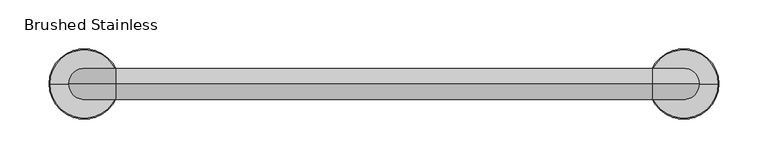
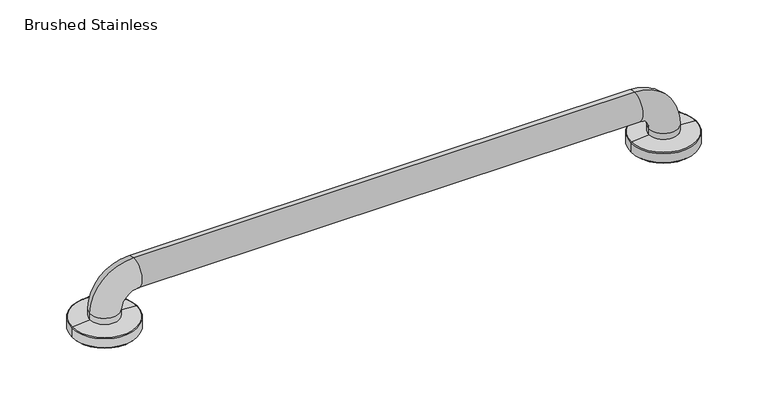
"""IFC4 building model written with IfcOpenShell, lengths in millimetres: furniture geometry, Grab_Bar-Kohler-Contemporary_K1456X : Brushed Stainless."""

import ifcopenshell
import ifcopenshell.guid

model = None  # the IFC model being written
_history = None  # IfcOwnerHistory: only IFC2X3 demands one
_inside = {}  # id of a spatial element -> (the spatial element, [elements in it])
_under = {}  # id of a project, library or spatial element -> (it, [spatial elements below it])
_declared = {}  # id of a project -> (the project, [libraries it declares])
_typed = {}  # id of a type object -> (the type object, [elements of that type])
_made_of = {}  # id of a material, layer set ... -> (it, [elements and type objects made of it])


def new_model(schema):
    """Start an empty IFC model of exactly this schema.

    Asked for "IFC4X3", IfcOpenShell would pick the latest addendum, in which some entities
    have other attributes; the version numbers below select the first issue.
    IFC2X3 requires an IfcOwnerHistory on every rooted entity: one is made here for all.
    """
    global model, _history
    if schema == "IFC4X3":
        model = ifcopenshell.file(schema_version=(4, 3, 0, 0))
    else:
        model = ifcopenshell.file(schema=schema)
    _inside.clear()
    _under.clear()
    _declared.clear()
    _typed.clear()
    _made_of.clear()
    _history = None
    if model.schema == "IFC2X3":
        org = make("IfcOrganization", Name="unknown")
        user = make(
            "IfcPersonAndOrganization",
            ThePerson=make("IfcPerson", FamilyName="unknown"),
            TheOrganization=org,
        )
        app = make(
            "IfcApplication",
            ApplicationDeveloper=org,
            Version="unknown",
            ApplicationFullName="unknown",
            ApplicationIdentifier="unknown",
        )
        _history = make(
            "IfcOwnerHistory",
            OwningUser=user,
            OwningApplication=app,
            ChangeAction="ADDED",
            CreationDate=0,
        )
    return model


def make(cls, **values):
    """One entity of the class cls with the attributes given. An attribute that is None is left unset."""
    return model.create_entity(
        cls, **{name: value for name, value in values.items() if value is not None}
    )


def rooted(cls, **values):
    """An entity with a GlobalId (a new one), such as an element, a storey or a relation."""
    return make(cls, GlobalId=ifcopenshell.guid.new(), OwnerHistory=_history, **values)


def si_unit(unit_type, name, prefix=None):
    """IfcSIUnit, for example si_unit("LENGTHUNIT", "METRE", prefix="MILLI")."""
    return make("IfcSIUnit", UnitType=unit_type, Prefix=prefix, Name=name)


def assignment(units):
    """IfcUnitAssignment: the units of a project."""
    return None if units is None else make("IfcUnitAssignment", Units=units)


def point(xyz):
    """IfcCartesianPoint."""
    return None if xyz is None else make("IfcCartesianPoint", Coordinates=xyz)


def direction(xyz):
    """IfcDirection."""
    return None if xyz is None else make("IfcDirection", DirectionRatios=xyz)


def frame(location, z_axis=None, x_axis=None):
    """IfcAxis2Placement3D, a coordinate frame: its origin and axes. An axis left out is left unset."""
    return make(
        "IfcAxis2Placement3D",
        Location=point(location),
        Axis=direction(z_axis),
        RefDirection=direction(x_axis),
    )


def origin():
    """The frame at (0, 0, 0) with its axes left unset."""
    return frame((0.0, 0.0, 0.0))


def place(relative_to, where):
    """IfcLocalPlacement: puts the frame where relative to a parent placement (None: the world)."""
    return make(
        "IfcLocalPlacement", PlacementRelTo=relative_to, RelativePlacement=where
    )


def context(
    kind, dimensions, precision=None, world=None, true_north=None, identifier=None
):
    """IfcGeometricRepresentationContext, for example the 3D "Model" context."""
    return make(
        "IfcGeometricRepresentationContext",
        ContextIdentifier=identifier,
        ContextType=kind,
        CoordinateSpaceDimension=dimensions,
        Precision=precision,
        WorldCoordinateSystem=world,
        TrueNorth=true_north,
    )


def project(units=None, contexts=None):
    """IfcProject with its units and contexts."""
    return rooted(
        "IfcProject",
        Name="project",
        RepresentationContexts=contexts,
        UnitsInContext=assignment(units),
    )


def spatial(cls, under=None, at=None, **own):
    """A site, building, storey or space (cls), placed at a placement, below another one or the project."""
    s = rooted(cls, ObjectPlacement=at, **own)
    if under is not None:
        _under.setdefault(under.id(), (under, []))[1].append(s)
    return s


def polyline(points):
    """IfcPolyline through the points."""
    return make("IfcPolyline", Points=[point(p) for p in points])


def circle_curve(where, radius):
    """IfcCircle in the frame where."""
    return make("IfcCircle", Position=where, Radius=radius)


def ellipse_curve(where, semi_axis1, semi_axis2):
    """IfcEllipse in the frame where."""
    return make(
        "IfcEllipse", Position=where, SemiAxis1=semi_axis1, SemiAxis2=semi_axis2
    )


def trimmed(basis, trim1, trim2, sense, master):
    """IfcTrimmedCurve: the piece of a basis curve between two trims."""
    return make(
        "IfcTrimmedCurve",
        BasisCurve=basis,
        Trim1=trim1,
        Trim2=trim2,
        SenseAgreement=sense,
        MasterRepresentation=master,
    )


def shape(context_of_items, identifier, shape_type, items):
    """IfcShapeRepresentation: the items that make up one representation, for example the "Body"."""
    return make(
        "IfcShapeRepresentation",
        ContextOfItems=context_of_items,
        RepresentationIdentifier=identifier,
        RepresentationType=shape_type,
        Items=items,
    )


def source(mapping_origin, context_of_items, identifier, shape_type, items):
    """IfcRepresentationMap: a shape defined once, which mapped items show again and again."""
    return make(
        "IfcRepresentationMap",
        MappingOrigin=mapping_origin,
        MappedRepresentation=shape(context_of_items, identifier, shape_type, items),
    )


def transform(
    local_origin,
    x_axis=None,
    y_axis=None,
    z_axis=None,
    scale=None,
    scale2=None,
    scale3=None,
    uniform=True,
):
    """IfcCartesianTransformationOperator3D, or its non-uniform kind. x_axis, y_axis, z_axis: its Axis1, 2, 3."""
    if uniform:
        return make(
            "IfcCartesianTransformationOperator3D",
            Axis1=direction(x_axis),
            Axis2=direction(y_axis),
            LocalOrigin=point(local_origin),
            Scale=scale,
            Axis3=direction(z_axis),
        )
    return make(
        "IfcCartesianTransformationOperator3DnonUniform",
        Axis1=direction(x_axis),
        Axis2=direction(y_axis),
        LocalOrigin=point(local_origin),
        Scale=scale,
        Axis3=direction(z_axis),
        Scale2=scale2,
        Scale3=scale3,
    )


def mapped(mapping_source, mapping_target):
    """IfcMappedItem: shows the shape of a source again, moved by a transform."""
    return make(
        "IfcMappedItem", MappingSource=mapping_source, MappingTarget=mapping_target
    )


def made_of(thing, what):
    """Note that an element or type object is made of a material, layer set ...; save() writes the relation."""
    if what is not None:
        _made_of.setdefault(what.id(), (what, []))[1].append(thing)
    return thing


def element(
    cls,
    number,
    at=None,
    inside=None,
    cuts=None,
    type_object=None,
    material=None,
    context=None,
    identifier="Body",
    shape_type=None,
    held_by="IfcProductDefinitionShape",
    body=None,
    shapes=None,
    **own,
):
    """One element of the class cls, such as IfcWall. Its Tag is "e" and its number.

    at: its placement. inside: the storey or other place that contains it. cuts: it is an
    opening in that element (IfcRelVoidsElement). A single representation is given by context,
    identifier, shape_type and body (its items); several are given by shapes. held_by: the class
    of the entity that holds the representations. save() writes the other relations.
    """
    e = rooted(cls, Tag="e%d" % number, ObjectPlacement=at, **own)
    if body is not None:
        shapes = [shape(context, identifier, shape_type, body)]
    if shapes is not None:
        e.Representation = make(held_by, Representations=shapes)
    if inside is not None:
        _inside.setdefault(inside.id(), (inside, []))[1].append(e)
    if cuts is not None:
        rooted(
            "IfcRelVoidsElement", RelatingBuildingElement=cuts, RelatedOpeningElement=e
        )
    if type_object is not None:
        _typed.setdefault(type_object.id(), (type_object, []))[1].append(e)
    return made_of(e, material)


def aggregate(whole, parts):
    """IfcRelAggregates: a whole, such as a stair, and the parts it consists of."""
    return rooted("IfcRelAggregates", RelatingObject=whole, RelatedObjects=parts)


def save(model, path):
    """Write the relations noted so far, then the file.

    IfcRelAggregates (storeys below a building ...), IfcRelContainedInSpatialStructure (elements
    in a storey), IfcRelDefinesByType, IfcRelAssociatesMaterial and IfcRelDeclares: one each for
    every whole, place, type object, material and project.
    """
    for whole, parts in _under.values():
        aggregate(whole, parts)
    for where, things in _inside.values():
        rooted(
            "IfcRelContainedInSpatialStructure",
            RelatedElements=things,
            RelatingStructure=where,
        )
    for kind, things in _typed.values():
        rooted("IfcRelDefinesByType", RelatedObjects=things, RelatingType=kind)
    for what, things in _made_of.values():
        rooted("IfcRelAssociatesMaterial", RelatedObjects=things, RelatingMaterial=what)
    for by, libraries in _declared.values():
        rooted("IfcRelDeclares", RelatingContext=by, RelatedDefinitions=libraries)
    model.write(path)


def plane_surface(at):
    """IfcPlane: the flat surface through the origin of the frame at, square to its z axis."""
    return make("IfcPlane", Position=at)


def cylinder_surface(at, radius):
    """IfcCylindricalSurface: all points at the distance radius from the z axis of the frame at."""
    return make("IfcCylindricalSurface", Position=at, Radius=radius)


def revolved_surface(curve, axis_point, axis_direction):
    """IfcSurfaceOfRevolution: the curve turned about the line through axis_point along axis_direction."""
    return make(
        "IfcSurfaceOfRevolution",
        SweptCurve=make("IfcArbitraryOpenProfileDef", ProfileType="CURVE", Curve=curve),
        AxisPosition=make("IfcAxis1Placement", Location=point(axis_point), Axis=direction(axis_direction)),
    )


def advanced_brep(points, edges, surfaces, faces):
    """IfcAdvancedBrep: a solid bounded by faces that lie on surfaces and meet in shared edges.

    An edge is (start, end): straight between two places in points (the first is 0);
    or (start, end, curve); or (start, end, curve, False) where it runs against its curve.
    A face is (place in surfaces, loops), or (place, loops, False) where it looks against
    its surface's normal. A loop lists edges by number (the first is 1), with a minus sign
    where the edge is run from its end to its start. The first loop is the outer one.
    """
    corners = [point(p) for p in points]
    vertices = [make("IfcVertexPoint", VertexGeometry=c) for c in corners]
    made = []
    for start, end, *more in edges:
        made.append(
            make(
                "IfcEdgeCurve",
                EdgeStart=vertices[start],
                EdgeEnd=vertices[end],
                EdgeGeometry=more[0] if more else make("IfcPolyline", Points=[corners[start], corners[end]]),
                SameSense=more[1] if len(more) > 1 else True,
            )
        )
    hull = []
    for where, loops, *sense in faces:
        bounds = []
        for j, loop in enumerate(loops):
            ring = [make("IfcOrientedEdge", EdgeElement=made[abs(k) - 1], Orientation=k > 0) for k in loop]
            bounds.append(
                make(
                    "IfcFaceOuterBound" if j == 0 else "IfcFaceBound",
                    Bound=make("IfcEdgeLoop", EdgeList=ring),
                    Orientation=True,
                )
            )
        hull.append(make("IfcAdvancedFace", Bounds=bounds, FaceSurface=surfaces[where], SameSense=sense[0] if sense else True))
    return make("IfcAdvancedBrep", Outer=make("IfcClosedShell", CfsFaces=hull))


def brushed_stainless_1e49a3ae(model_context):
    return source(origin(), model_context, "Body", "AdvancedBrep", [
        advanced_brep(
        [(288.925, 0.0, 15.08125), (320.675, 0.0, 15.08125), (339.5910439, 0.0, 13.5506193), (270.0089561, 0.0, 13.5506193), (288.925, 0.0, 0.0), (320.675, 0.0, 0.0), (271.45615, 0.0, 0.0), (338.14385, 0.0, 0.0), (269.0749, 0.0, 2.38125), (340.5251, 0.0, 2.38125), (269.0749, 0.0, 12.5379293), (340.5251, 0.0, 12.5379293)],
        [
            (0, 1, circle_curve(frame((304.8, 0.0, 15.08125), z_axis=(0.0, 0.0, -1.0), x_axis=(1.0, 0.0, 0.0)), 15.875)),
            (1, 2),
            (2, 3, circle_curve(frame((304.8, 0.0, 13.5506193), z_axis=(0.0, 0.0, 1.0), x_axis=(1.0, 0.0, 0.0)), 34.7910439)),
            (3, 0),
            (1, 0, circle_curve(frame((304.8, 0.0, 15.08125), z_axis=(0.0, 0.0, -1.0), x_axis=(1.0, 0.0, 0.0)), 15.875)),
            (3, 2, circle_curve(frame((304.8, 0.0, 13.5506193), z_axis=(0.0, 0.0, 1.0), x_axis=(1.0, 0.0, 0.0)), 34.7910439)),
            (4, 5, circle_curve(frame((304.8, 0.0, 0.0), z_axis=(0.0, 0.0, -1.0), x_axis=(1.0, 0.0, 0.0)), 15.875)),
            (5, 1),
            (0, 4),
            (5, 4, circle_curve(frame((304.8, 0.0, 0.0), z_axis=(0.0, 0.0, -1.0), x_axis=(1.0, 0.0, 0.0)), 15.875)),
            (6, 7, circle_curve(frame((304.8, 0.0, 0.0), z_axis=(0.0, 0.0, -1.0), x_axis=(1.0, 0.0, 0.0)), 33.34385)),
            (7, 5),
            (4, 6),
            (7, 6, circle_curve(frame((304.8, 0.0, 0.0), z_axis=(0.0, 0.0, -1.0), x_axis=(1.0, 0.0, 0.0)), 33.34385)),
            (8, 9, circle_curve(frame((304.8, 0.0, 2.38125), z_axis=(0.0, 0.0, -1.0), x_axis=(1.0, 0.0, 0.0)), 35.7251)),
            (9, 7),
            (6, 8),
            (9, 8, circle_curve(frame((304.8, 0.0, 2.38125), z_axis=(0.0, 0.0, -1.0), x_axis=(1.0, 0.0, 0.0)), 35.7251)),
            (10, 11, circle_curve(frame((304.8, 0.0, 12.5379293), z_axis=(0.0, 0.0, -1.0), x_axis=(1.0, 0.0, 0.0)), 35.7251)),
            (11, 9),
            (8, 10),
            (11, 10, circle_curve(frame((304.8, 0.0, 12.5379293), z_axis=(0.0, 0.0, -1.0), x_axis=(1.0, 0.0, 0.0)), 35.7251)),
            (2, 11, circle_curve(frame((339.5091, 0.0, 12.5379293), z_axis=(0.0, 1.0, 0.0), x_axis=(1.0, 0.0, 0.0)), 1.016)),
            (10, 3, circle_curve(frame((270.0909, 0.0, 12.5379293), z_axis=(0.0, 1.0, 0.0), x_axis=(-1.0, 0.0, 0.0)), 1.016)),
        ],
        [
            revolved_surface(polyline([(339.5910439, 0.0, 13.5506193), (320.675, 0.0, 15.08125)]), (304.8, 0.0, 136.525), (0.0, 0.0, 1.0)),
            revolved_surface(polyline([(320.675, 0.0, 15.081249999999997), (320.675, 0.0, 0.0)]), (304.8, 0.0, 136.525), (0.0, 0.0, 1.0)),
            plane_surface(frame((304.8, 0.0, 0.0), z_axis=(0.0, 0.0, -1.0), x_axis=(1.0, 0.0, 0.0))),
            revolved_surface(polyline([(338.14385, 0.0, 0.0), (340.5251, 0.0, 2.38125)]), (304.8, 0.0, 136.525), (0.0, 0.0, 1.0)),
            cylinder_surface(frame((304.8, 0.0, 136.525), z_axis=(0.0, 0.0, 1.0), x_axis=(1.0, 0.0, 0.0)), 35.7251),
            revolved_surface(trimmed(ellipse_curve(frame((339.5091, 0.0, 12.5379293), z_axis=(0.0, -1.0, 0.0), x_axis=(1.0, 0.0, 0.0)), 1.016, 1.016), [point((340.5251, 0.0, 12.5379293))], [point((339.5910439, 0.0, 13.5506193))], True, "CARTESIAN"), (304.8, 0.0, 136.525), (0.0, 0.0, 1.0)),
        ],
        [
            (0, [[1, 2, 3, 4]]),
            (0, [[5, -4, 6, -2]]),
            (1, [[7, 8, -1, 9]]),
            (1, [[10, -9, -5, -8]]),
            (2, [[11, 12, -7, 13]]),
            (2, [[14, -13, -10, -12]]),
            (3, [[15, 16, -11, 17]]),
            (3, [[18, -17, -14, -16]]),
            (4, [[19, 20, -15, 21]]),
            (4, [[22, -21, -18, -20]]),
            (5, [[-3, 23, -19, 24]]),
            (5, [[-6, -24, -22, -23]]),
        ],
    ),
        advanced_brep(
        [(-270.0089561, 0.0, 13.5506193), (-339.5910439, 0.0, 13.5506193), (-320.675, 0.0, 15.08125), (-288.925, 0.0, 15.08125), (-269.0749, 0.0, 2.38125), (-340.5251, 0.0, 2.38125), (-340.5251, 0.0, 12.5379293), (-269.0749, 0.0, 12.5379293), (-271.45615, 0.0, 0.0), (-338.14385, 0.0, 0.0), (-288.925, 0.0, 0.0), (-320.675, 0.0, 0.0)],
        [
            (0, 1, circle_curve(frame((-304.8, 0.0, 13.5506193), z_axis=(0.0, 0.0, 1.0), x_axis=(-1.0, 0.0, 0.0)), 34.7910439)),
            (1, 2),
            (2, 3, circle_curve(frame((-304.8, 0.0, 15.08125), z_axis=(0.0, 0.0, -1.0), x_axis=(-1.0, 0.0, 0.0)), 15.875)),
            (3, 0),
            (1, 0, circle_curve(frame((-304.8, 0.0, 13.5506193), z_axis=(0.0, 0.0, 1.0), x_axis=(-1.0, 0.0, 0.0)), 34.7910439)),
            (3, 2, circle_curve(frame((-304.8, 0.0, 15.08125), z_axis=(0.0, 0.0, -1.0), x_axis=(-1.0, 0.0, 0.0)), 15.875)),
            (4, 5, circle_curve(frame((-304.8, 0.0, 2.38125), z_axis=(0.0, 0.0, 1.0), x_axis=(-1.0, 0.0, 0.0)), 35.7251)),
            (5, 6),
            (6, 7, circle_curve(frame((-304.8, 0.0, 12.5379293), z_axis=(0.0, 0.0, -1.0), x_axis=(-1.0, 0.0, 0.0)), 35.7251)),
            (7, 4),
            (5, 4, circle_curve(frame((-304.8, 0.0, 2.38125), z_axis=(0.0, 0.0, 1.0), x_axis=(-1.0, 0.0, 0.0)), 35.7251)),
            (7, 6, circle_curve(frame((-304.8, 0.0, 12.5379293), z_axis=(0.0, 0.0, -1.0), x_axis=(-1.0, 0.0, 0.0)), 35.7251)),
            (8, 9, circle_curve(frame((-304.8, 0.0, 0.0), z_axis=(0.0, 0.0, 1.0), x_axis=(-1.0, 0.0, 0.0)), 33.34385)),
            (9, 5),
            (4, 8),
            (9, 8, circle_curve(frame((-304.8, 0.0, 0.0), z_axis=(0.0, 0.0, 1.0), x_axis=(-1.0, 0.0, 0.0)), 33.34385)),
            (10, 11, circle_curve(frame((-304.8, 0.0, 0.0), z_axis=(0.0, 0.0, 1.0), x_axis=(-1.0, 0.0, 0.0)), 15.875)),
            (11, 9),
            (8, 10),
            (11, 10, circle_curve(frame((-304.8, 0.0, 0.0), z_axis=(0.0, 0.0, 1.0), x_axis=(-1.0, 0.0, 0.0)), 15.875)),
            (2, 11),
            (10, 3),
            (6, 1, circle_curve(frame((-339.5091, 0.0, 12.5379293), z_axis=(0.0, 1.0, 0.0), x_axis=(1.0, 0.0, 0.0)), 1.016)),
            (0, 7, circle_curve(frame((-270.0909, 0.0, 12.5379293), z_axis=(0.0, 1.0, 0.0), x_axis=(-1.0, 0.0, 0.0)), 1.016)),
        ],
        [
            revolved_surface(polyline([(-320.675, 0.0, 15.08125), (-339.5910439, 0.0, 13.5506193)]), (-304.8, 0.0, 70.0128086), (0.0, 0.0, -1.0)),
            cylinder_surface(frame((-304.8, 0.0, 70.0128086), z_axis=(0.0, 0.0, -1.0), x_axis=(-1.0, 0.0, 0.0)), 35.7251),
            revolved_surface(polyline([(-340.5251, 0.0, 2.38125), (-338.14385, 0.0, 0.0)]), (-304.8, 0.0, 70.0128086), (0.0, 0.0, -1.0)),
            plane_surface(frame((-304.8, 0.0, 0.0), z_axis=(0.0, 0.0, -1.0), x_axis=(-1.0, 0.0, 0.0))),
            revolved_surface(polyline([(-320.675, 0.0, 0.0), (-320.675, 0.0, 15.081249999999997)]), (-304.8, 0.0, 70.0128086), (0.0, 0.0, -1.0)),
            revolved_surface(trimmed(ellipse_curve(frame((-339.5091, 0.0, 12.5379293), z_axis=(0.0, -1.0, 0.0), x_axis=(1.0, 0.0, 0.0)), 1.016, 1.016), [point((-339.5910439, 0.0, 13.5506193))], [point((-340.5251, 0.0, 12.5379293))], True, "CARTESIAN"), (-304.8, 0.0, 70.0128086), (0.0, 0.0, -1.0)),
        ],
        [
            (0, [[1, 2, 3, 4]]),
            (0, [[5, -4, 6, -2]]),
            (1, [[7, 8, 9, 10]]),
            (1, [[11, -10, 12, -8]]),
            (2, [[13, 14, -7, 15]]),
            (2, [[16, -15, -11, -14]]),
            (3, [[17, 18, -13, 19]]),
            (3, [[20, -19, -16, -18]]),
            (4, [[-3, 21, -17, 22]]),
            (4, [[-6, -22, -20, -21]]),
            (5, [[-9, 23, -1, 24]]),
            (5, [[-12, -24, -5, -23]]),
        ],
    ),
        advanced_brep(
        [(-288.925, 0.0, 0.0), (-320.675, 0.0, 0.0), (-288.925, 0.0, 22.225), (-320.675, 0.0, 22.225), (-273.05, 0.0, 69.85), (-273.05, 0.0, 38.1), (273.05, 0.0, 38.1), (273.05, 0.0, 69.85), (320.675, 0.0, 22.225), (288.925, 0.0, 22.225), (288.925, 0.0, 0.0), (320.675, 0.0, 0.0)],
        [
            (0, 1, circle_curve(frame((-304.8, 0.0, 0.0), z_axis=(0.0, 0.0, -1.0), x_axis=(-1.0, 0.0, 0.0)), 15.875)),
            (1, 0, circle_curve(frame((-304.8, 0.0, 0.0), z_axis=(0.0, 0.0, -1.0), x_axis=(-1.0, 0.0, 0.0)), 15.875)),
            (0, 2),
            (2, 3, circle_curve(frame((-304.8, 0.0, 22.225), z_axis=(0.0, 0.0, -1.0), x_axis=(-1.0, 0.0, 0.0)), 15.875)),
            (3, 1),
            (3, 2, circle_curve(frame((-304.8, 0.0, 22.225), z_axis=(0.0, 0.0, -1.0), x_axis=(-1.0, 0.0, 0.0)), 15.875)),
            (4, 3, circle_curve(frame((-273.05, 0.0, 22.225), z_axis=(0.0, -1.0, 0.0), x_axis=(-1.0, 0.0, 0.0)), 47.625)),
            (2, 5, circle_curve(frame((-273.05, 0.0, 22.225), z_axis=(0.0, 1.0, 0.0), x_axis=(-1.0, 0.0, 0.0)), 15.875)),
            (5, 4, circle_curve(frame((-273.05, 0.0, 53.975), z_axis=(-1.0, 0.0, 0.0), x_axis=(0.0, 0.0, 1.0)), 15.875)),
            (4, 5, circle_curve(frame((-273.05, 0.0, 53.975), z_axis=(-1.0, 0.0, 0.0), x_axis=(0.0, 0.0, 1.0)), 15.875)),
            (5, 6),
            (6, 7, circle_curve(frame((273.05, 0.0, 53.975), z_axis=(-1.0, 0.0, 0.0), x_axis=(0.0, 0.0, 1.0)), 15.875)),
            (7, 4),
            (7, 6, circle_curve(frame((273.05, 0.0, 53.975), z_axis=(-1.0, 0.0, 0.0), x_axis=(0.0, 0.0, 1.0)), 15.875)),
            (8, 7, circle_curve(frame((273.05, 0.0, 22.225), z_axis=(0.0, -1.0, 0.0), x_axis=(0.0, 0.0, 1.0)), 47.625)),
            (6, 9, circle_curve(frame((273.05, 0.0, 22.225), z_axis=(0.0, 1.0, 0.0), x_axis=(0.0, 0.0, 1.0)), 15.875)),
            (9, 8, circle_curve(frame((304.8, 0.0, 22.225), z_axis=(0.0, 0.0, 1.0), x_axis=(1.0, 0.0, 0.0)), 15.875)),
            (8, 9, circle_curve(frame((304.8, 0.0, 22.225), z_axis=(0.0, 0.0, 1.0), x_axis=(1.0, 0.0, 0.0)), 15.875)),
            (10, 11, circle_curve(frame((304.8, 0.0, 0.0), z_axis=(0.0, 0.0, -1.0), x_axis=(1.0, 0.0, 0.0)), 15.875)),
            (11, 10, circle_curve(frame((304.8, 0.0, 0.0), z_axis=(0.0, 0.0, -1.0), x_axis=(1.0, 0.0, 0.0)), 15.875)),
            (9, 10),
            (11, 8),
        ],
        [
            plane_surface(frame((-304.8, 0.0, 0.0), z_axis=(0.0, 0.0, -1.0), x_axis=(0.0, -1.0, 0.0))),
            cylinder_surface(frame((-304.8, 0.0, 0.0), z_axis=(0.0, 0.0, -1.0), x_axis=(-1.0, 0.0, 0.0)), 15.875),
            revolved_surface(trimmed(ellipse_curve(frame((-304.8, 0.0, 22.225), z_axis=(0.0, 0.0, -1.0), x_axis=(-1.0, 0.0, 0.0)), 15.875, 15.875), [point((-288.925, 0.0, 22.225))], [point((-320.675, 0.0, 22.225))], True, "CARTESIAN"), (-273.05, 0.0, 22.225), (0.0, 1.0, 0.0)),
            revolved_surface(trimmed(ellipse_curve(frame((-304.8, 0.0, 22.225), z_axis=(0.0, 0.0, -1.0), x_axis=(-1.0, 0.0, 0.0)), 15.875, 15.875), [point((-320.675, 0.0, 22.225))], [point((-288.925, 0.0, 22.225))], True, "CARTESIAN"), (-273.05, 0.0, 22.225), (0.0, 1.0, 0.0)),
            cylinder_surface(frame((-273.05, 0.0, 53.975), z_axis=(-1.0, 0.0, 0.0), x_axis=(0.0, 0.0, 1.0)), 15.875),
            revolved_surface(trimmed(ellipse_curve(frame((273.05, 0.0, 53.975), z_axis=(-1.0, 0.0, 0.0), x_axis=(0.0, 0.0, 1.0)), 15.875, 15.875), [point((273.05, 0.0, 38.1))], [point((273.05, 0.0, 69.85))], True, "CARTESIAN"), (273.05, 0.0, 22.225), (0.0, 1.0, 0.0)),
            revolved_surface(trimmed(ellipse_curve(frame((273.05, 0.0, 53.975), z_axis=(-1.0, 0.0, 0.0), x_axis=(0.0, 0.0, 1.0)), 15.875, 15.875), [point((273.05, 0.0, 69.85))], [point((273.05, 0.0, 38.1))], True, "CARTESIAN"), (273.05, 0.0, 22.225), (0.0, 1.0, 0.0)),
            plane_surface(frame((304.8, 0.0, 0.0), z_axis=(0.0, 0.0, -1.0), x_axis=(0.0, -1.0, 0.0))),
            cylinder_surface(frame((304.8, 0.0, 22.225), z_axis=(0.0, 0.0, 1.0), x_axis=(1.0, 0.0, 0.0)), 15.875),
        ],
        [
            (0, [[1, 2]]),
            (1, [[-1, 3, 4, 5]]),
            (1, [[-2, -5, 6, -3]]),
            (2, [[7, -4, 8, 9]]),
            (3, [[-8, -6, -7, 10]]),
            (4, [[-9, 11, 12, 13]]),
            (4, [[-10, -13, 14, -11]]),
            (5, [[15, -12, 16, 17]]),
            (6, [[-16, -14, -15, 18]]),
            (7, [[19, 20]]),
            (8, [[-17, 21, -20, 22]]),
            (8, [[-18, -22, -19, -21]]),
        ],
    ),
    ])


if __name__ == "__main__":
    model = new_model("IFC4")
    model_context = context("Model", 3, world=origin())
    ifc_project = project(units=[si_unit("LENGTHUNIT", "METRE", prefix="MILLI")], contexts=[model_context])
    site = spatial("IfcSite", under=ifc_project)
    building = spatial("IfcBuilding", under=site)
    placement = place(None, origin())
    brushed_stainless_shape = brushed_stainless_1e49a3ae(model_context)
    element("IfcFurniture", 1, ObjectType="Grab_Bar-Kohler-Contemporary_K1456X : Brushed Stainless", at=placement, inside=building, context=model_context, shape_type="MappedRepresentation", body=[
        mapped(brushed_stainless_shape, transform((0.0, 0.0, 0.0), x_axis=(1.0, 0.0, 0.0), y_axis=(0.0, 1.0, 0.0), z_axis=(0.0, 0.0, 1.0))),
    ])
    save(model, "model.ifc")

# Revit data of these elements
# Type "Grab_Bar-Kohler-Contemporary_K1456X : Brushed Stainless"
#   zz Text 1 [instance default] = "Available"
#   URL = "http://www.us.kohler.com/us/"
#   Product Page URL = "http://www.us.kohler.com/us/catalog/productDetails.jsp?productNumber=14567"
#   Part Number [instance default] = "K-14560-BS"
#   Part Description [instance default] = "12 Inch Brushed Stainless Steel Contemporary Grab Bar"
#   Model Disclaimer = "Contact Kohler Company For More Information"
#   Model = "See Part Number"
#   Manufacturer = "Kohler Company"
#   Family Version = "1.0"
#   Equipment Number [instance default] = ""
#   Equipment Abbreviation = "GB"
#   Description = "See Part Description"
#   Date Modified = "September 25, 2014"
#   Date Created = "September 25, 2014"
#   Copyright = "Copyright ©2014 Kohler Company"
#   zz Length 7 [instance default] = 6.35 mm
#   zz Length 6 [instance default] = 6.35 mm
#   zz Length 5 [instance default] = 6.35 mm
#   zz Length 4 = 71.45 mm
#   zz Length 3 = 53.975 mm
#   zz Length 2 [instance default] = 376.25 mm
#   zz Length 1 = 35.725 mm
#   Width [instance default] = 69.85 mm
#   Length [instance default] = 376.25 mm
#   Height [instance default] = 71.45 mm
#   Default Elevation = 1219.20 mm
#   zz YesNo 1 [instance default] = no
#   zz Integer 2 [instance default] = 1
#   zz Integer 1 = 4
#   Length is 54 Inches [instance default] = no
#   Length is 48 Inches [instance default] = no
#   Length is 42 Inches [instance default] = no
#   Length is 36 Inches [instance default] = no
#   Length is 32 Inches [instance default] = no
#   Length is 24 Inches [instance default] = no
#   Length is 18 Inches [instance default] = no
#   Length is 12 Inches [instance default] = yes
#   Product Material = Metal - Kohler - Brushed Stainless
# Element 1 (IfcFurniture, "Grab_Bar-Kohler-Contemporary_K1456X : Brushed Stainless")
#   Part Number = "K-14562-BS"
#   Part Description = "24 Inch Brushed Stainless Steel Contemporary Grab Bar"
#   zz Length 2 = 681.05 mm
#   Length = 681.05 mm
#   zz Integer 2 = 3
#   Length is 24 Inches = yes
#   Length is 12 Inches = no
#   Materials on its faces: "Metal - Kohler - Brushed Stainless"
# Materials
#   "Metal - Kohler - Brushed Stainless": class "Miscellaneous", colour RGB 189 187 185, transparency 0
